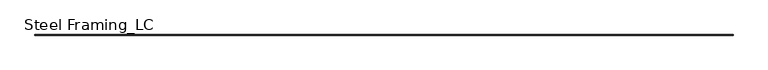
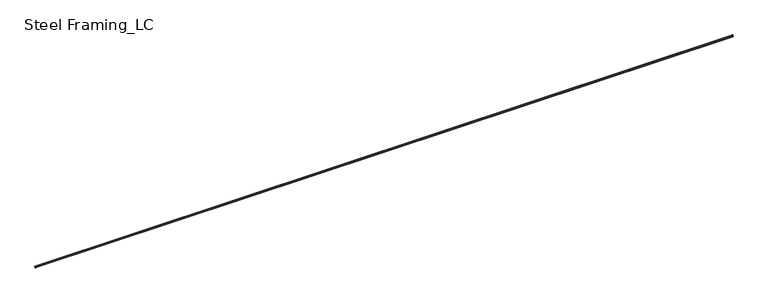
"""IFC4 building model written with IfcOpenShell, lengths in millimetres: beam geometry, Steel Framing_LC : H_SB_AR_S00_LC-150x75x25x3.2."""

from ifc_helpers import new_model, si_unit, point, frame, frame_2d, origin, place, context, project, spatial, polyline, circle_curve, trimmed, segment, composite_curve, outline, extrude, source, transform, mapped, element, save


def steel_framing_lc_01a803ec(model_context):
    return source(origin(), model_context, "Body", "SweptSolid", [
        extrude(outline(composite_curve([segment(polyline([(18.6, 67.0), (18.6, -67.0)]), True, "CONTINUOUS"), segment(trimmed(circle_curve(frame_2d((10.6, -67.0)), 8.0), [point((18.6, -67.0))], [point((10.6, -75.0))], False, "CARTESIAN"), True, "CONTINUOUS"), segment(polyline([(10.6, -75.0), (-48.4, -75.0)]), True, "CONTINUOUS"), segment(trimmed(circle_curve(frame_2d((-48.4, -67.0)), 8.0), [point((-48.4, -75.0))], [point((-56.4, -67.0))], False, "CARTESIAN"), True, "CONTINUOUS"), segment(polyline([(-56.4, -67.0), (-56.4, -50.0), (-53.2, -50.0), (-53.2, -67.0)]), True, "CONTINUOUS"), segment(trimmed(circle_curve(frame_2d((-48.4, -67.0)), 4.8), [point((-53.2, -67.0))], [point((-48.4, -71.8))], True, "CARTESIAN"), True, "CONTINUOUS"), segment(polyline([(-48.4, -71.8), (10.6, -71.8)]), True, "CONTINUOUS"), segment(trimmed(circle_curve(frame_2d((10.6, -67.0)), 4.8), [point((10.6, -71.8))], [point((15.4, -67.0))], True, "CARTESIAN"), True, "CONTINUOUS"), segment(polyline([(15.4, -67.0), (15.4, 67.0)]), True, "CONTINUOUS"), segment(trimmed(circle_curve(frame_2d((10.6, 67.0)), 4.8), [point((15.4, 67.0))], [point((10.6, 71.8))], True, "CARTESIAN"), True, "CONTINUOUS"), segment(polyline([(10.6, 71.8), (-48.4, 71.8)]), True, "CONTINUOUS"), segment(trimmed(circle_curve(frame_2d((-48.4, 67.0)), 4.8), [point((-48.4, 71.8))], [point((-53.2, 67.0))], True, "CARTESIAN"), True, "CONTINUOUS"), segment(polyline([(-53.2, 67.0), (-53.2, 50.0), (-56.4, 50.0), (-56.4, 67.0)]), True, "CONTINUOUS"), segment(trimmed(circle_curve(frame_2d((-48.4, 67.0)), 8.0), [point((-56.4, 67.0))], [point((-48.4, 75.0))], False, "CARTESIAN"), True, "CONTINUOUS"), segment(polyline([(-48.4, 75.0), (10.6, 75.0)]), True, "CONTINUOUS"), segment(trimmed(circle_curve(frame_2d((10.6, 67.0)), 8.0), [point((10.6, 75.0))], [point((18.6, 67.0))], False, "CARTESIAN"), True, "CONTINUOUS")], self_intersect=False)), frame((-39375.0, 0.0, 0.0), z_axis=(1.0, 0.0, 0.0), x_axis=(0.0, 1.0, 0.0)), (0.0, 0.0, 1.0), 78750.0),
    ])


if __name__ == "__main__":
    model = new_model("IFC4")
    model_context = context("Model", 3, world=origin())
    ifc_project = project(units=[si_unit("LENGTHUNIT", "METRE", prefix="MILLI")], contexts=[model_context])
    site = spatial("IfcSite", under=ifc_project)
    building = spatial("IfcBuilding", under=site)
    placement = place(None, origin())
    steel_framing_lc_shape = steel_framing_lc_01a803ec(model_context)
    element("IfcBeam", 1, ObjectType="Steel Framing_LC : H_SB_AR_S00_LC-150x75x25x3.2", at=placement, inside=building, context=model_context, shape_type="MappedRepresentation", body=[
        mapped(steel_framing_lc_shape, transform((0.0, 0.0, 0.0), x_axis=(1.0, 0.0, 0.0), y_axis=(0.0, 1.0, 0.0), z_axis=(0.0, 0.0, 1.0))),
    ])
    save(model, "model.ifc")

# Revit data of these elements
# Type "Steel Framing_LC : H_SB_AR_S00_LC-150x75x25x3.2"
#   Type Comments = "SECONDARY"
#   Type Mark = "GIRTH"
#   H_SectionID = "LC-150x75x25x3.2"
#   r = 4.8 mm
#   d = 25 mm
#   R = 8 mm
#   Perimeter = 0.70 m²/m
#   Nominal Weight = 10.30 kgf/m
#   Length [instance default] = 1000 mm
#   b = 75 mm
#   h = 150 mm
#   tw = 3.2 mm
#   x = 18.6 mm
#   A = 1.00 m²
#   Structural Material [instance default] = Steel, 45-345
#   Assembly Code = ""
# Element 1 (IfcBeam, "Steel Framing_LC : H_SB_AR_S00_LC-150x75x25x3.2")
#   Materials on its faces: "Steel, 45-345"
# Materials
#   "Steel, 45-345": class "Metal", colour RGB 189 187 185, transparency 0, Description = "Steel 345 MPa", Cost = 0
